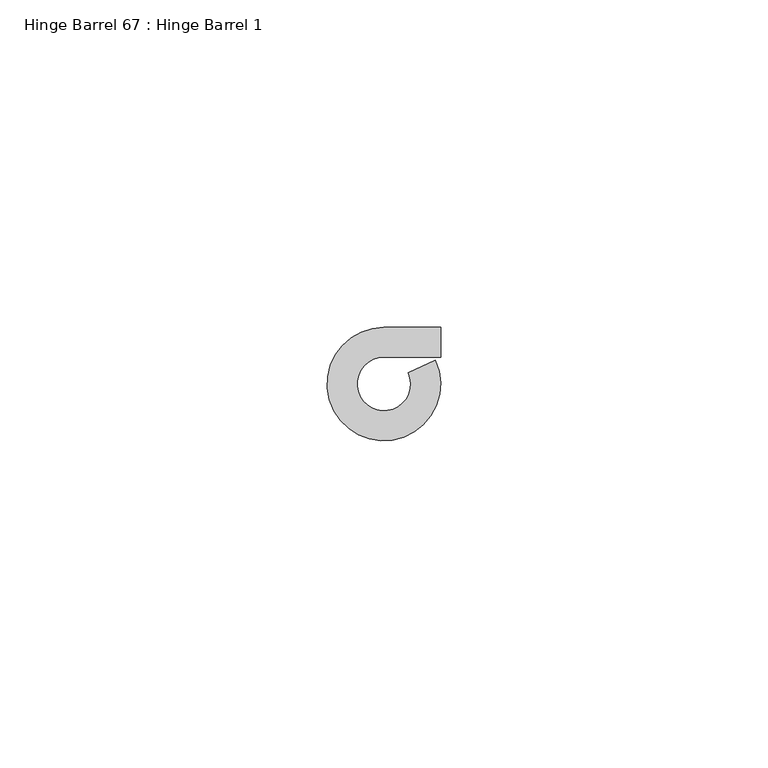
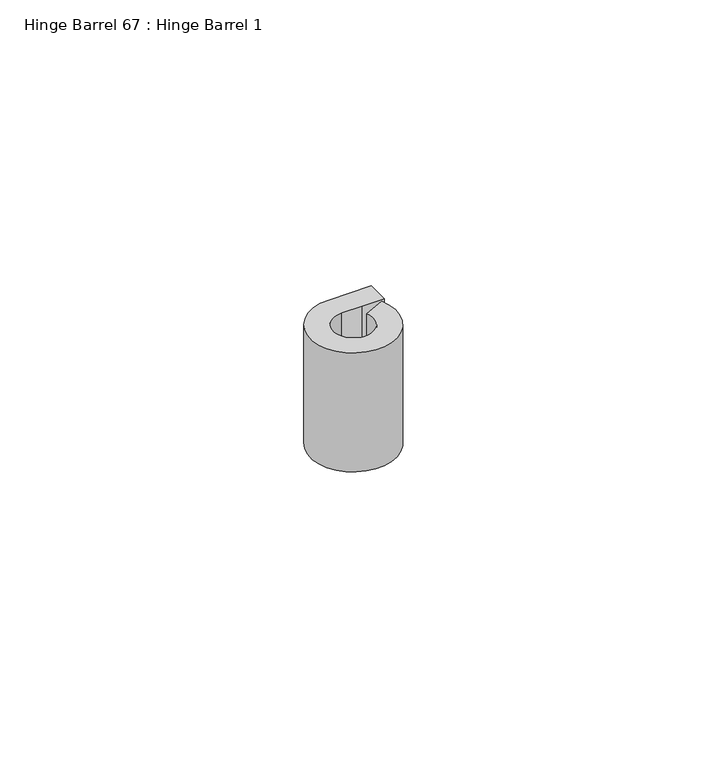
"""IFC4 building model written with IfcOpenShell, lengths in millimetres: proxy geometry, Hinge Barrel 67 : Hinge Barrel 1."""

from ifc_helpers import new_model, si_unit, point, frame, frame_2d, origin, place, context, project, spatial, polyline, circle_curve, trimmed, segment, composite_curve, outline, extrude, source, transform, mapped, element, save


def hinge_barrel_67_hinge_barrel_1_2f8cd32d(model_context):
    return source(origin(), model_context, "Body", "SweptSolid", [
        extrude(outline(composite_curve([segment(polyline([(587323.2214739, -536306.2758841), (587319.1320739, -536306.2758841)]), True, "CONTINUOUS"), segment(trimmed(circle_curve(frame_2d((587319.1320739, -536310.3652841)), 4.0894), [point((587319.1320739, -536306.2758841))], [point((587322.8436736, -536308.6485371))], True, "CARTESIAN"), True, "CONTINUOUS"), segment(polyline([(587322.8436736, -536308.6485371), (587326.986084, -536306.7325249)]), True, "CONTINUOUS"), segment(trimmed(circle_curve(frame_2d((587319.1320739, -536310.3652841)), 8.6534625), [point((587326.986084, -536306.7325249))], [point((587319.1320739, -536301.7118216))], False, "CARTESIAN"), True, "CONTINUOUS"), segment(polyline([(587319.1320739, -536301.7118216), (587327.7934739, -536301.7118216), (587327.7934739, -536306.2758841), (587323.2214739, -536306.2758841)]), True, "CONTINUOUS")], self_intersect=False)), frame((0.0, 0.0, 1123.95), z_axis=(0.0, 0.0, 1.0), x_axis=(1.0, 0.0, 0.0)), (0.0, 0.0, 1.0), 25.4),
    ])


if __name__ == "__main__":
    model = new_model("IFC4")
    model_context = context("Model", 3, world=origin())
    ifc_project = project(units=[si_unit("LENGTHUNIT", "METRE", prefix="MILLI")], contexts=[model_context])
    site = spatial("IfcSite", under=ifc_project)
    building = spatial("IfcBuilding", under=site)
    placement = place(None, origin())
    hinge_barrel_67_hinge_barrel_1_shape = hinge_barrel_67_hinge_barrel_1_2f8cd32d(model_context)
    element("IfcBuildingElementProxy", 1, Name="Hinge Barrel 67 : Hinge Barrel 1", ObjectType="Hinge Barrel 67 : Hinge Barrel 1", at=placement, inside=building, context=model_context, shape_type="MappedRepresentation", body=[
        mapped(hinge_barrel_67_hinge_barrel_1_shape, transform((0.0, 0.0, 0.0), x_axis=(1.0, 0.0, 0.0), y_axis=(0.0, 1.0, 0.0), z_axis=(0.0, 0.0, 1.0))),
    ])
    save(model, "model.ifc")

# Revit data of these elements
# Element 1 (IfcBuildingElementProxy, "Hinge Barrel 67 : Hinge Barrel 1")
#   Materials on its faces: "6\"X6\" WELD-ON STL BUTT HINGE"
# Materials
#   "6\"X6\" WELD-ON STL BUTT HINGE": class "Metal", colour RGB 189 187 185, transparency 0, Description = "Carbon steel", Cost = 0
